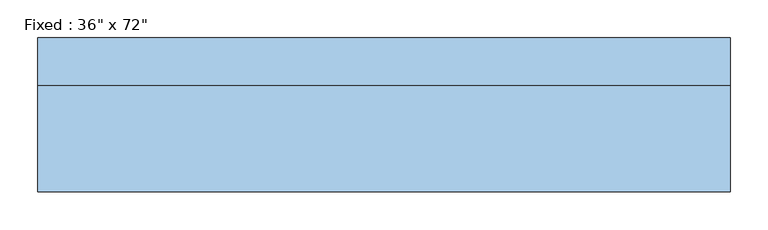
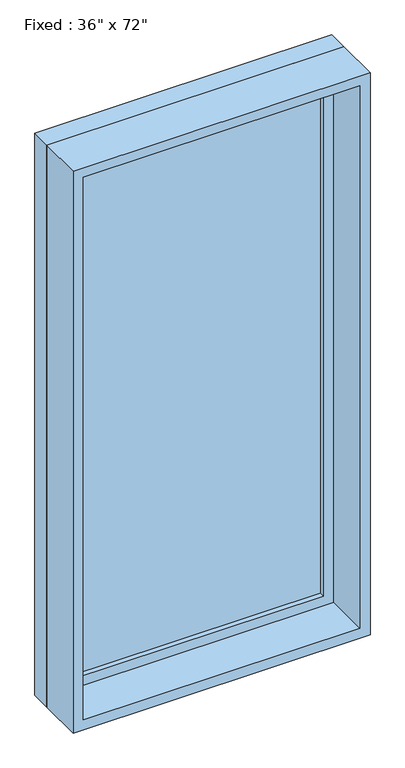
"""IFC4 building model written with IfcOpenShell, lengths in millimetres: window geometry."""

import ifcopenshell
import ifcopenshell.guid

model = None  # the IFC model being written
_history = None  # IfcOwnerHistory: only IFC2X3 demands one
_inside = {}  # id of a spatial element -> (the spatial element, [elements in it])
_under = {}  # id of a project, library or spatial element -> (it, [spatial elements below it])
_declared = {}  # id of a project -> (the project, [libraries it declares])
_typed = {}  # id of a type object -> (the type object, [elements of that type])
_made_of = {}  # id of a material, layer set ... -> (it, [elements and type objects made of it])


def new_model(schema):
    """Start an empty IFC model of exactly this schema.

    Asked for "IFC4X3", IfcOpenShell would pick the latest addendum, in which some entities
    have other attributes; the version numbers below select the first issue.
    IFC2X3 requires an IfcOwnerHistory on every rooted entity: one is made here for all.
    """
    global model, _history
    if schema == "IFC4X3":
        model = ifcopenshell.file(schema_version=(4, 3, 0, 0))
    else:
        model = ifcopenshell.file(schema=schema)
    _inside.clear()
    _under.clear()
    _declared.clear()
    _typed.clear()
    _made_of.clear()
    _history = None
    if model.schema == "IFC2X3":
        org = make("IfcOrganization", Name="unknown")
        user = make(
            "IfcPersonAndOrganization",
            ThePerson=make("IfcPerson", FamilyName="unknown"),
            TheOrganization=org,
        )
        app = make(
            "IfcApplication",
            ApplicationDeveloper=org,
            Version="unknown",
            ApplicationFullName="unknown",
            ApplicationIdentifier="unknown",
        )
        _history = make(
            "IfcOwnerHistory",
            OwningUser=user,
            OwningApplication=app,
            ChangeAction="ADDED",
            CreationDate=0,
        )
    return model


def make(cls, **values):
    """One entity of the class cls with the attributes given. An attribute that is None is left unset."""
    return model.create_entity(
        cls, **{name: value for name, value in values.items() if value is not None}
    )


def rooted(cls, **values):
    """An entity with a GlobalId (a new one), such as an element, a storey or a relation."""
    return make(cls, GlobalId=ifcopenshell.guid.new(), OwnerHistory=_history, **values)


def si_unit(unit_type, name, prefix=None):
    """IfcSIUnit, for example si_unit("LENGTHUNIT", "METRE", prefix="MILLI")."""
    return make("IfcSIUnit", UnitType=unit_type, Prefix=prefix, Name=name)


def assignment(units):
    """IfcUnitAssignment: the units of a project."""
    return None if units is None else make("IfcUnitAssignment", Units=units)


def point(xyz):
    """IfcCartesianPoint."""
    return None if xyz is None else make("IfcCartesianPoint", Coordinates=xyz)


def direction(xyz):
    """IfcDirection."""
    return None if xyz is None else make("IfcDirection", DirectionRatios=xyz)


def frame(location, z_axis=None, x_axis=None):
    """IfcAxis2Placement3D, a coordinate frame: its origin and axes. An axis left out is left unset."""
    return make(
        "IfcAxis2Placement3D",
        Location=point(location),
        Axis=direction(z_axis),
        RefDirection=direction(x_axis),
    )


def origin():
    """The frame at (0, 0, 0) with its axes left unset."""
    return frame((0.0, 0.0, 0.0))


def place(relative_to, where):
    """IfcLocalPlacement: puts the frame where relative to a parent placement (None: the world)."""
    return make(
        "IfcLocalPlacement", PlacementRelTo=relative_to, RelativePlacement=where
    )


def context(
    kind, dimensions, precision=None, world=None, true_north=None, identifier=None
):
    """IfcGeometricRepresentationContext, for example the 3D "Model" context."""
    return make(
        "IfcGeometricRepresentationContext",
        ContextIdentifier=identifier,
        ContextType=kind,
        CoordinateSpaceDimension=dimensions,
        Precision=precision,
        WorldCoordinateSystem=world,
        TrueNorth=true_north,
    )


def project(units=None, contexts=None):
    """IfcProject with its units and contexts."""
    return rooted(
        "IfcProject",
        Name="project",
        RepresentationContexts=contexts,
        UnitsInContext=assignment(units),
    )


def spatial(cls, under=None, at=None, **own):
    """A site, building, storey or space (cls), placed at a placement, below another one or the project."""
    s = rooted(cls, ObjectPlacement=at, **own)
    if under is not None:
        _under.setdefault(under.id(), (under, []))[1].append(s)
    return s


def polyline(points):
    """IfcPolyline through the points."""
    return make("IfcPolyline", Points=[point(p) for p in points])


def outline(outer, holes=None, kind="AREA"):
    """IfcArbitraryClosedProfileDef: a profile drawn as a closed curve; with holes, ...WithVoids."""
    if holes is None:
        return make("IfcArbitraryClosedProfileDef", ProfileType=kind, OuterCurve=outer)
    return make(
        "IfcArbitraryProfileDefWithVoids",
        ProfileType=kind,
        OuterCurve=outer,
        InnerCurves=holes,
    )


def extrude(swept, where, along, depth):
    """IfcExtrudedAreaSolid: the profile swept, set in the frame where, extruded along a direction by depth."""
    return make(
        "IfcExtrudedAreaSolid",
        SweptArea=swept,
        Position=where,
        ExtrudedDirection=direction(along),
        Depth=depth,
    )


def shape(context_of_items, identifier, shape_type, items):
    """IfcShapeRepresentation: the items that make up one representation, for example the "Body"."""
    return make(
        "IfcShapeRepresentation",
        ContextOfItems=context_of_items,
        RepresentationIdentifier=identifier,
        RepresentationType=shape_type,
        Items=items,
    )


def source(mapping_origin, context_of_items, identifier, shape_type, items):
    """IfcRepresentationMap: a shape defined once, which mapped items show again and again."""
    return make(
        "IfcRepresentationMap",
        MappingOrigin=mapping_origin,
        MappedRepresentation=shape(context_of_items, identifier, shape_type, items),
    )


def transform(
    local_origin,
    x_axis=None,
    y_axis=None,
    z_axis=None,
    scale=None,
    scale2=None,
    scale3=None,
    uniform=True,
):
    """IfcCartesianTransformationOperator3D, or its non-uniform kind. x_axis, y_axis, z_axis: its Axis1, 2, 3."""
    if uniform:
        return make(
            "IfcCartesianTransformationOperator3D",
            Axis1=direction(x_axis),
            Axis2=direction(y_axis),
            LocalOrigin=point(local_origin),
            Scale=scale,
            Axis3=direction(z_axis),
        )
    return make(
        "IfcCartesianTransformationOperator3DnonUniform",
        Axis1=direction(x_axis),
        Axis2=direction(y_axis),
        LocalOrigin=point(local_origin),
        Scale=scale,
        Axis3=direction(z_axis),
        Scale2=scale2,
        Scale3=scale3,
    )


def mapped(mapping_source, mapping_target):
    """IfcMappedItem: shows the shape of a source again, moved by a transform."""
    return make(
        "IfcMappedItem", MappingSource=mapping_source, MappingTarget=mapping_target
    )


def made_of(thing, what):
    """Note that an element or type object is made of a material, layer set ...; save() writes the relation."""
    if what is not None:
        _made_of.setdefault(what.id(), (what, []))[1].append(thing)
    return thing


def element(
    cls,
    number,
    at=None,
    inside=None,
    cuts=None,
    type_object=None,
    material=None,
    context=None,
    identifier="Body",
    shape_type=None,
    held_by="IfcProductDefinitionShape",
    body=None,
    shapes=None,
    **own,
):
    """One element of the class cls, such as IfcWall. Its Tag is "e" and its number.

    at: its placement. inside: the storey or other place that contains it. cuts: it is an
    opening in that element (IfcRelVoidsElement). A single representation is given by context,
    identifier, shape_type and body (its items); several are given by shapes. held_by: the class
    of the entity that holds the representations. save() writes the other relations.
    """
    e = rooted(cls, Tag="e%d" % number, ObjectPlacement=at, **own)
    if body is not None:
        shapes = [shape(context, identifier, shape_type, body)]
    if shapes is not None:
        e.Representation = make(held_by, Representations=shapes)
    if inside is not None:
        _inside.setdefault(inside.id(), (inside, []))[1].append(e)
    if cuts is not None:
        rooted(
            "IfcRelVoidsElement", RelatingBuildingElement=cuts, RelatedOpeningElement=e
        )
    if type_object is not None:
        _typed.setdefault(type_object.id(), (type_object, []))[1].append(e)
    return made_of(e, material)


def aggregate(whole, parts):
    """IfcRelAggregates: a whole, such as a stair, and the parts it consists of."""
    return rooted("IfcRelAggregates", RelatingObject=whole, RelatedObjects=parts)


def save(model, path):
    """Write the relations noted so far, then the file.

    IfcRelAggregates (storeys below a building ...), IfcRelContainedInSpatialStructure (elements
    in a storey), IfcRelDefinesByType, IfcRelAssociatesMaterial and IfcRelDeclares: one each for
    every whole, place, type object, material and project.
    """
    for whole, parts in _under.values():
        aggregate(whole, parts)
    for where, things in _inside.values():
        rooted(
            "IfcRelContainedInSpatialStructure",
            RelatedElements=things,
            RelatingStructure=where,
        )
    for kind, things in _typed.values():
        rooted("IfcRelDefinesByType", RelatedObjects=things, RelatingType=kind)
    for what, things in _made_of.values():
        rooted("IfcRelAssociatesMaterial", RelatedObjects=things, RelatingMaterial=what)
    for by, libraries in _declared.values():
        rooted("IfcRelDeclares", RelatingContext=by, RelatedDefinitions=libraries)
    model.write(path)


def window_9a779fa2(model_context):
    return source(origin(), model_context, "Body", "SweptSolid", [
        extrude(outline(polyline([(355.6, 53.975), (-431.8, 53.975), (-431.8, 66.675), (355.6, 66.675), (355.6, 53.975)])), frame((0.0, 0.0, 368.3), z_axis=(0.0, 0.0, 1.0), x_axis=(1.0, 0.0, 0.0)), (0.0, 0.0, 1.0), 1701.8),
        extrude(outline(polyline([(2114.55, -476.25), (323.85, -476.25), (323.85, 400.05), (2114.55, 400.05), (2114.55, -476.25)]), holes=[polyline([(2070.1, -431.8), (2070.1, 355.6), (368.3, 355.6), (368.3, -431.8), (2070.1, -431.8)])]), frame((0.0, 38.1, 0.0), z_axis=(0.0, 1.0, 0.0), x_axis=(0.0, 0.0, 1.0)), (0.0, 0.0, 1.0), 44.45),
        extrude(outline(polyline([(2133.6, -495.3), (304.8, -495.3), (304.8, 419.1), (2133.6, 419.1), (2133.6, -495.3)]), holes=[polyline([(2101.85, -463.55), (2101.85, 387.35), (336.55, 387.35), (336.55, -463.55), (2101.85, -463.55)])]), frame((0.0, -101.6, 0.0), z_axis=(0.0, 1.0, 0.0), x_axis=(0.0, 0.0, 1.0)), (0.0, 0.0, 1.0), 139.7),
        extrude(outline(polyline([(2133.6, 419.1), (2133.6, -495.3), (304.8, -495.3), (304.8, 419.1), (2133.6, 419.1)]), holes=[polyline([(2114.55, 400.05), (323.85, 400.05), (323.85, -476.25), (2114.55, -476.25), (2114.55, 400.05)])]), frame((0.0, 38.1, 0.0), z_axis=(0.0, 1.0, 0.0), x_axis=(0.0, 0.0, 1.0)), (0.0, 0.0, 1.0), 63.5),
    ])


if __name__ == "__main__":
    model = new_model("IFC4")
    model_context = context("Model", 3, world=origin())
    ifc_project = project(units=[si_unit("LENGTHUNIT", "METRE", prefix="MILLI")], contexts=[model_context])
    site = spatial("IfcSite", under=ifc_project)
    building = spatial("IfcBuilding", under=site)
    placement = place(None, origin())
    window_shape = window_9a779fa2(model_context)
    element("IfcWindow", 1, ObjectType="Fixed : 36\" x 72\"", at=placement, inside=building, context=model_context, shape_type="MappedRepresentation", body=[
        mapped(window_shape, transform((0.0, 0.0, 0.0), x_axis=(1.0, 0.0, 0.0), y_axis=(0.0, 1.0, 0.0), z_axis=(0.0, 0.0, 1.0))),
    ])
    save(model, "model.ifc")

# Revit data of these elements
# Type "Fixed : 36\" x 72\""
#   Type Mark = "9"
#   Construction Type Id = "GSP4R"
#   Assembly Code = "B2020100"
#   Analytic Construction = "1/8 in Pilkington single glazing"
#   Visual Light Transmittance = 0.9
#   Solar Heat Gain Coefficient = 0.78
#   Heat Transfer Coefficient (U) = 3.6886 W/(m²·K)
#   Height = 6' - 0"
#   Default Sill Height = 1' - 0"
#   Width = 3' - 0"
#   Window Inset = 0' - 0 3/4"
#   Glass Pane Material = Glass
#   Sash Material = Sash
#   Wall Closure = (empty or 0)
# Element 1 (IfcWindow, "Fixed : 36\" x 72\"")
#   Materials on its faces: "Sash", "Glass"
# Materials
#   "Glass": class "Glass", colour RGB 0 128 192, transparency 0.75, Description = "Soda Lime Glass", Cost = 0
#   "Sash": class "Wood", colour RGB 224 178 126, transparency 0, Cost = 0
